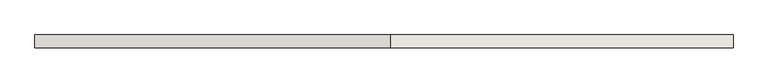
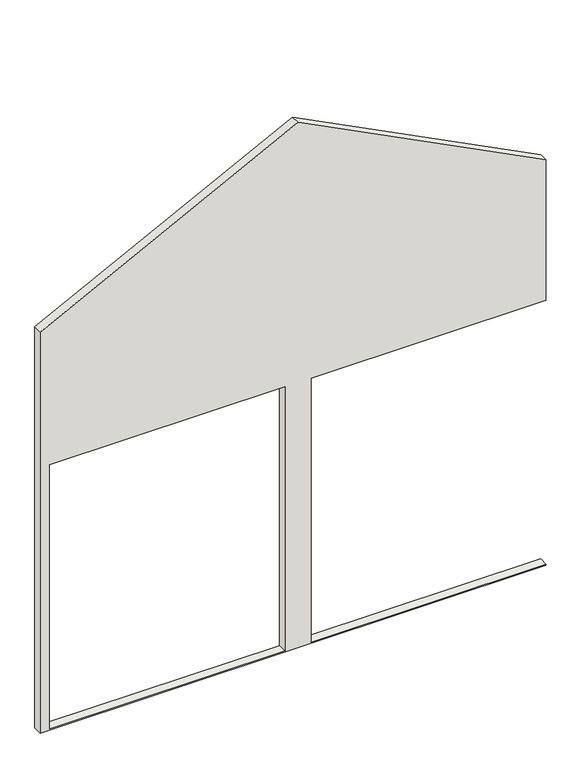
"""IFC4 building model written with IfcOpenShell, lengths in millimetres: wall geometry, 0_3d_modell."""

from ifc_helpers import new_model, si_unit, frame, origin, place, context, project, spatial, polyline, outline, extrude, source, transform, mapped, element, save


def wall_6a45402e(model_context):
    return source(origin(), model_context, "Body", "SweptSolid", [
        extrude(outline(polyline([(10.0, 3875.0), (10.0, 2075.0), (2145.0, 2075.0), (2145.0, 3875.0), (3283.5797924, 3875.0), (4251.6781465, 1975.0), (3245.3653837, 0.0), (0.0, 0.0), (0.0, 3875.0), (10.0, 3875.0)]), holes=[polyline([(2145.0, 1875.0), (10.0, 1875.0), (10.0, 75.0), (2145.0, 75.0), (2145.0, 1875.0)])]), frame((0.0, 0.0, 0.0), z_axis=(0.0, 1.0, 0.0), x_axis=(0.0, 0.0, 1.0)), (0.0, 0.0, 1.0), 70.0),
    ])


if __name__ == "__main__":
    model = new_model("IFC4")
    model_context = context("Model", 3, world=origin())
    ifc_project = project(units=[si_unit("LENGTHUNIT", "METRE", prefix="MILLI")], contexts=[model_context])
    site = spatial("IfcSite", under=ifc_project)
    building = spatial("IfcBuilding", under=site)
    placement = place(None, origin())
    wall_shape = wall_6a45402e(model_context)
    element("IfcWall", 1, ObjectType="0_3d_modell", at=placement, inside=building, context=model_context, shape_type="MappedRepresentation", body=[
        mapped(wall_shape, transform((0.0, 0.0, 0.0), x_axis=(1.0, 0.0, 0.0), y_axis=(0.0, 1.0, 0.0), z_axis=(0.0, 0.0, 1.0))),
    ])
    save(model, "model.ifc")

# Revit data of these elements
# Element 1 (IfcWall, "0_3d_modell")
#   Materials on its faces: "Glass_Simple"
# Materials
#   "Glass_Simple": class "Unassigned", colour RGB 255 255 255, transparency 0.9
